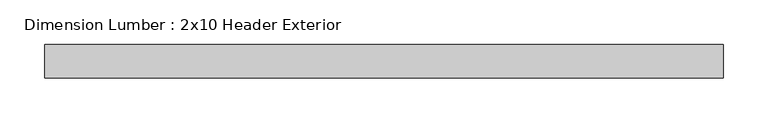
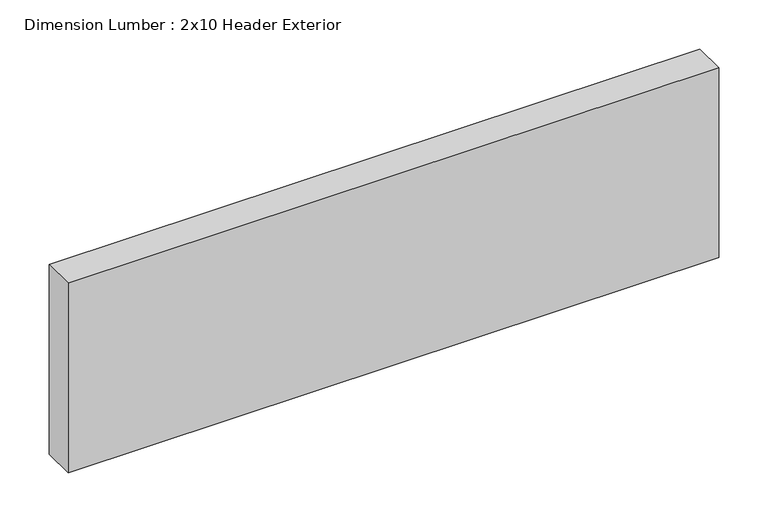
"""IFC4 building model written with IfcOpenShell, lengths in millimetres: beam geometry, Dimension Lumber : 2x10 Header Exterior."""

from ifc_helpers import new_model, si_unit, frame, origin, place, context, project, spatial, polyline, outline, extrude, source, transform, mapped, element, save


def dimension_lumber_2x10_header_exterior_5ef0ce1b(model_context):
    return source(origin(), model_context, "Body", "SweptSolid", [
        extrude(outline(polyline([(468.709375, -19.05), (-293.290625, -19.05), (-293.290625, 19.05), (468.709375, 19.05), (468.709375, -19.05)])), frame((0.0, 0.0, -117.475), z_axis=(0.0, 0.0, 1.0), x_axis=(1.0, 0.0, 0.0)), (0.0, 0.0, 1.0), 234.95),
    ])


if __name__ == "__main__":
    model = new_model("IFC4")
    model_context = context("Model", 3, world=origin())
    ifc_project = project(units=[si_unit("LENGTHUNIT", "METRE", prefix="MILLI")], contexts=[model_context])
    site = spatial("IfcSite", under=ifc_project)
    building = spatial("IfcBuilding", under=site)
    placement = place(None, origin())
    dimension_lumber_2x10_header_exterior_shape = dimension_lumber_2x10_header_exterior_5ef0ce1b(model_context)
    element("IfcBeam", 1, ObjectType="Dimension Lumber : 2x10 Header Exterior", at=placement, inside=building, context=model_context, shape_type="MappedRepresentation", body=[
        mapped(dimension_lumber_2x10_header_exterior_shape, transform((0.0, 0.0, 0.0), x_axis=(1.0, 0.0, 0.0), y_axis=(0.0, 1.0, 0.0), z_axis=(0.0, 0.0, 1.0))),
    ])
    save(model, "model.ifc")

# Revit data of these elements
# Type "Dimension Lumber : 2x10 Header Exterior"
#   Assembly Code = "B10"
#   A = 0.0963889 SF
#   Length [instance default] = 5' - 0"
#   b = 0' - 1 1/2"
#   d = 0' - 9 1/4"
#   Structural Material [instance default] = Softwood, Lumber
# Element 1 (IfcBeam, "Dimension Lumber : 2x10 Header Exterior")
#   Structural Material = Douglas Fir #2
#   Materials on its faces: "Douglas Fir #2"
# Materials
#   "Softwood, Lumber": class "Wood", colour RGB 223 192 134, transparency 0, Description = "Pinus Echinata", Cost = 0
#   "Douglas Fir #2": class "Wood", colour RGB 223 192 134, transparency 0, Description = "Pinus Echinata", Cost = 0
